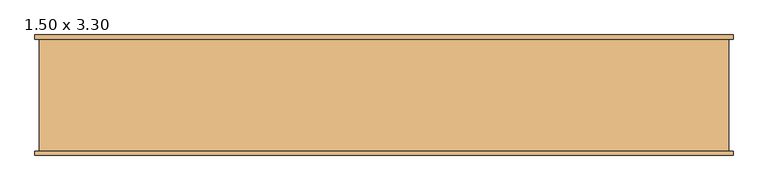
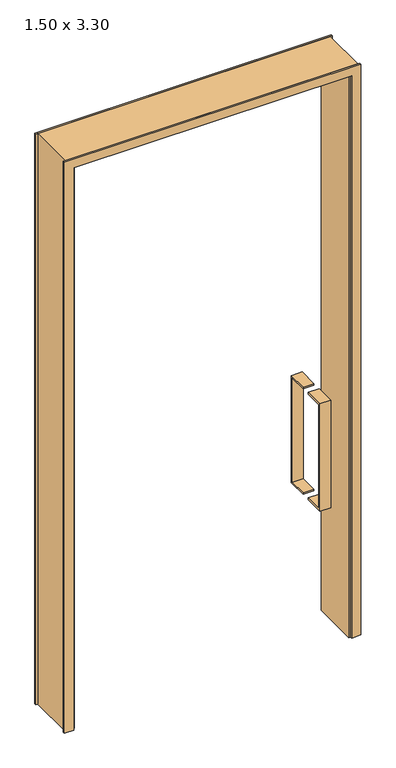
"""IFC4 building model written with IfcOpenShell, lengths in millimetres: door geometry, .CC_ND 300 PORTA PIVOTANTE_COM BANDEIRA_COM EXTENSÃO : 1.50 x 3.30."""

import ifcopenshell
import ifcopenshell.guid

model = None  # the IFC model being written
_history = None  # IfcOwnerHistory: only IFC2X3 demands one
_inside = {}  # id of a spatial element -> (the spatial element, [elements in it])
_under = {}  # id of a project, library or spatial element -> (it, [spatial elements below it])
_declared = {}  # id of a project -> (the project, [libraries it declares])
_typed = {}  # id of a type object -> (the type object, [elements of that type])
_made_of = {}  # id of a material, layer set ... -> (it, [elements and type objects made of it])


def new_model(schema):
    """Start an empty IFC model of exactly this schema.

    Asked for "IFC4X3", IfcOpenShell would pick the latest addendum, in which some entities
    have other attributes; the version numbers below select the first issue.
    IFC2X3 requires an IfcOwnerHistory on every rooted entity: one is made here for all.
    """
    global model, _history
    if schema == "IFC4X3":
        model = ifcopenshell.file(schema_version=(4, 3, 0, 0))
    else:
        model = ifcopenshell.file(schema=schema)
    _inside.clear()
    _under.clear()
    _declared.clear()
    _typed.clear()
    _made_of.clear()
    _history = None
    if model.schema == "IFC2X3":
        org = make("IfcOrganization", Name="unknown")
        user = make(
            "IfcPersonAndOrganization",
            ThePerson=make("IfcPerson", FamilyName="unknown"),
            TheOrganization=org,
        )
        app = make(
            "IfcApplication",
            ApplicationDeveloper=org,
            Version="unknown",
            ApplicationFullName="unknown",
            ApplicationIdentifier="unknown",
        )
        _history = make(
            "IfcOwnerHistory",
            OwningUser=user,
            OwningApplication=app,
            ChangeAction="ADDED",
            CreationDate=0,
        )
    return model


def make(cls, **values):
    """One entity of the class cls with the attributes given. An attribute that is None is left unset."""
    return model.create_entity(
        cls, **{name: value for name, value in values.items() if value is not None}
    )


def rooted(cls, **values):
    """An entity with a GlobalId (a new one), such as an element, a storey or a relation."""
    return make(cls, GlobalId=ifcopenshell.guid.new(), OwnerHistory=_history, **values)


def si_unit(unit_type, name, prefix=None):
    """IfcSIUnit, for example si_unit("LENGTHUNIT", "METRE", prefix="MILLI")."""
    return make("IfcSIUnit", UnitType=unit_type, Prefix=prefix, Name=name)


def assignment(units):
    """IfcUnitAssignment: the units of a project."""
    return None if units is None else make("IfcUnitAssignment", Units=units)


def point(xyz):
    """IfcCartesianPoint."""
    return None if xyz is None else make("IfcCartesianPoint", Coordinates=xyz)


def direction(xyz):
    """IfcDirection."""
    return None if xyz is None else make("IfcDirection", DirectionRatios=xyz)


def frame(location, z_axis=None, x_axis=None):
    """IfcAxis2Placement3D, a coordinate frame: its origin and axes. An axis left out is left unset."""
    return make(
        "IfcAxis2Placement3D",
        Location=point(location),
        Axis=direction(z_axis),
        RefDirection=direction(x_axis),
    )


def origin():
    """The frame at (0, 0, 0) with its axes left unset."""
    return frame((0.0, 0.0, 0.0))


def place(relative_to, where):
    """IfcLocalPlacement: puts the frame where relative to a parent placement (None: the world)."""
    return make(
        "IfcLocalPlacement", PlacementRelTo=relative_to, RelativePlacement=where
    )


def context(
    kind, dimensions, precision=None, world=None, true_north=None, identifier=None
):
    """IfcGeometricRepresentationContext, for example the 3D "Model" context."""
    return make(
        "IfcGeometricRepresentationContext",
        ContextIdentifier=identifier,
        ContextType=kind,
        CoordinateSpaceDimension=dimensions,
        Precision=precision,
        WorldCoordinateSystem=world,
        TrueNorth=true_north,
    )


def project(units=None, contexts=None):
    """IfcProject with its units and contexts."""
    return rooted(
        "IfcProject",
        Name="project",
        RepresentationContexts=contexts,
        UnitsInContext=assignment(units),
    )


def spatial(cls, under=None, at=None, **own):
    """A site, building, storey or space (cls), placed at a placement, below another one or the project."""
    s = rooted(cls, ObjectPlacement=at, **own)
    if under is not None:
        _under.setdefault(under.id(), (under, []))[1].append(s)
    return s


def polyline(points):
    """IfcPolyline through the points."""
    return make("IfcPolyline", Points=[point(p) for p in points])


def outline(outer, holes=None, kind="AREA"):
    """IfcArbitraryClosedProfileDef: a profile drawn as a closed curve; with holes, ...WithVoids."""
    if holes is None:
        return make("IfcArbitraryClosedProfileDef", ProfileType=kind, OuterCurve=outer)
    return make(
        "IfcArbitraryProfileDefWithVoids",
        ProfileType=kind,
        OuterCurve=outer,
        InnerCurves=holes,
    )


def extrude(swept, where, along, depth):
    """IfcExtrudedAreaSolid: the profile swept, set in the frame where, extruded along a direction by depth."""
    return make(
        "IfcExtrudedAreaSolid",
        SweptArea=swept,
        Position=where,
        ExtrudedDirection=direction(along),
        Depth=depth,
    )


def shape(context_of_items, identifier, shape_type, items):
    """IfcShapeRepresentation: the items that make up one representation, for example the "Body"."""
    return make(
        "IfcShapeRepresentation",
        ContextOfItems=context_of_items,
        RepresentationIdentifier=identifier,
        RepresentationType=shape_type,
        Items=items,
    )


def source(mapping_origin, context_of_items, identifier, shape_type, items):
    """IfcRepresentationMap: a shape defined once, which mapped items show again and again."""
    return make(
        "IfcRepresentationMap",
        MappingOrigin=mapping_origin,
        MappedRepresentation=shape(context_of_items, identifier, shape_type, items),
    )


def transform(
    local_origin,
    x_axis=None,
    y_axis=None,
    z_axis=None,
    scale=None,
    scale2=None,
    scale3=None,
    uniform=True,
):
    """IfcCartesianTransformationOperator3D, or its non-uniform kind. x_axis, y_axis, z_axis: its Axis1, 2, 3."""
    if uniform:
        return make(
            "IfcCartesianTransformationOperator3D",
            Axis1=direction(x_axis),
            Axis2=direction(y_axis),
            LocalOrigin=point(local_origin),
            Scale=scale,
            Axis3=direction(z_axis),
        )
    return make(
        "IfcCartesianTransformationOperator3DnonUniform",
        Axis1=direction(x_axis),
        Axis2=direction(y_axis),
        LocalOrigin=point(local_origin),
        Scale=scale,
        Axis3=direction(z_axis),
        Scale2=scale2,
        Scale3=scale3,
    )


def mapped(mapping_source, mapping_target):
    """IfcMappedItem: shows the shape of a source again, moved by a transform."""
    return make(
        "IfcMappedItem", MappingSource=mapping_source, MappingTarget=mapping_target
    )


def made_of(thing, what):
    """Note that an element or type object is made of a material, layer set ...; save() writes the relation."""
    if what is not None:
        _made_of.setdefault(what.id(), (what, []))[1].append(thing)
    return thing


def element(
    cls,
    number,
    at=None,
    inside=None,
    cuts=None,
    type_object=None,
    material=None,
    context=None,
    identifier="Body",
    shape_type=None,
    held_by="IfcProductDefinitionShape",
    body=None,
    shapes=None,
    **own,
):
    """One element of the class cls, such as IfcWall. Its Tag is "e" and its number.

    at: its placement. inside: the storey or other place that contains it. cuts: it is an
    opening in that element (IfcRelVoidsElement). A single representation is given by context,
    identifier, shape_type and body (its items); several are given by shapes. held_by: the class
    of the entity that holds the representations. save() writes the other relations.
    """
    e = rooted(cls, Tag="e%d" % number, ObjectPlacement=at, **own)
    if body is not None:
        shapes = [shape(context, identifier, shape_type, body)]
    if shapes is not None:
        e.Representation = make(held_by, Representations=shapes)
    if inside is not None:
        _inside.setdefault(inside.id(), (inside, []))[1].append(e)
    if cuts is not None:
        rooted(
            "IfcRelVoidsElement", RelatingBuildingElement=cuts, RelatedOpeningElement=e
        )
    if type_object is not None:
        _typed.setdefault(type_object.id(), (type_object, []))[1].append(e)
    return made_of(e, material)


def aggregate(whole, parts):
    """IfcRelAggregates: a whole, such as a stair, and the parts it consists of."""
    return rooted("IfcRelAggregates", RelatingObject=whole, RelatedObjects=parts)


def save(model, path):
    """Write the relations noted so far, then the file.

    IfcRelAggregates (storeys below a building ...), IfcRelContainedInSpatialStructure (elements
    in a storey), IfcRelDefinesByType, IfcRelAssociatesMaterial and IfcRelDeclares: one each for
    every whole, place, type object, material and project.
    """
    for whole, parts in _under.values():
        aggregate(whole, parts)
    for where, things in _inside.values():
        rooted(
            "IfcRelContainedInSpatialStructure",
            RelatedElements=things,
            RelatingStructure=where,
        )
    for kind, things in _typed.values():
        rooted("IfcRelDefinesByType", RelatedObjects=things, RelatingType=kind)
    for what, things in _made_of.values():
        rooted("IfcRelAssociatesMaterial", RelatedObjects=things, RelatingMaterial=what)
    for by, libraries in _declared.values():
        rooted("IfcRelDeclares", RelatingContext=by, RelatedDefinitions=libraries)
    model.write(path)


def door_1_50_x_3_30_2c3f3e4b(model_context):
    return source(origin(), model_context, "Body", "SweptSolid", [
        extrude(outline(polyline([(0.0, -810.0), (0.0, -760.0), (3250.0, -760.0), (3250.0, 760.0), (0.0, 760.0), (0.0, 810.0), (3300.0, 810.0), (3300.0, -810.0), (0.0, -810.0)])), frame((0.0, -139.9, 0.0), z_axis=(0.0, 1.0, 0.0), x_axis=(0.0, 0.0, 1.0)), (0.0, 0.0, 1.0), 10.0),
        extrude(outline(polyline([(0.0, 760.0), (0.0, 810.0), (3300.0, 810.0), (3300.0, -810.0), (0.0, -810.0), (0.0, -760.0), (3250.0, -760.0), (3250.0, 760.0), (0.0, 760.0)])), frame((0.0, 129.9, 0.0), z_axis=(0.0, 1.0, 0.0), x_axis=(0.0, 0.0, 1.0)), (0.0, 0.0, 1.0), 10.0),
        extrude(outline(polyline([(0.0, -800.0), (0.0, -750.0), (3250.0, -750.0), (3250.0, 750.0), (0.0, 750.0), (0.0, 800.0), (3300.0, 800.0), (3300.0, -800.0), (0.0, -800.0)])), frame((0.0, -129.9, 0.0), z_axis=(0.0, 1.0, 0.0), x_axis=(0.0, 0.0, 1.0)), (0.0, 0.0, 1.0), 259.8),
        extrude(outline(polyline([(-25.0, 1410.0), (-25.0, 1400.0), (-125.0, 1400.0), (-125.0, 800.0), (-25.0, 800.0), (-25.0, 790.0), (-135.0, 790.0), (-135.0, 1410.0), (-25.0, 1410.0)])), frame((590.0, 0.0, 0.0), z_axis=(1.0, 0.0, 0.0), x_axis=(0.0, 1.0, 0.0)), (0.0, 0.0, 1.0), 60.0),
        extrude(outline(polyline([(25.0, 1400.0), (25.0, 1410.0), (135.0, 1410.0), (135.0, 790.0), (25.0, 790.0), (25.0, 800.0), (125.0, 800.0), (125.0, 1400.0), (25.0, 1400.0)])), frame((590.0, 0.0, 0.0), z_axis=(1.0, 0.0, 0.0), x_axis=(0.0, 1.0, 0.0)), (0.0, 0.0, 1.0), 60.0),
    ])


if __name__ == "__main__":
    model = new_model("IFC4")
    model_context = context("Model", 3, world=origin())
    ifc_project = project(units=[si_unit("LENGTHUNIT", "METRE", prefix="MILLI")], contexts=[model_context])
    site = spatial("IfcSite", under=ifc_project)
    building = spatial("IfcBuilding", under=site)
    placement = place(None, origin())
    door_1_50_x_3_30_shape = door_1_50_x_3_30_2c3f3e4b(model_context)
    element("IfcDoor", 1, ObjectType=".CC_ND 300 PORTA PIVOTANTE_COM BANDEIRA_COM EXTENSÃO : 1.50 x 3.30", at=placement, inside=building, context=model_context, shape_type="MappedRepresentation", body=[
        mapped(door_1_50_x_3_30_shape, transform((0.0, 0.0, 0.0), x_axis=(1.0, 0.0, 0.0), y_axis=(0.0, 1.0, 0.0), z_axis=(0.0, 0.0, 1.0))),
    ])
    save(model, "model.ifc")

# Revit data of these elements
# Type ".CC_ND 300 PORTA PIVOTANTE_COM BANDEIRA_COM EXTENSÃO : 1.50 x 3.30"
#   Type Mark = "151"
#   Analytic Construction = "<None>"
#   Pivot = 0.10 m
#   Largura moldura = 0.05 m
#   Rough Width = 1.60 m
#   Extensão do acabamento interior [instance default] = 0.00 m
#   Extensão do acabamento exterior [instance default] = 0.00 m
#   Espessura moldura = 0.01 m
#   Espessura batente = 0.05 m
#   Thickness = 0.05 m
#   Rough Height = 3.30 m
#   Altura bandeira = 1.15 m
#   Height = 2.10 m
#   Width = 1.50 m
#   Puxador interno [instance default] = yes
#   Puxador externo [instance default] = yes
#   Número de ripas da porta = 4
#   Moldura interna [instance default] = yes
#   Moldura externa [instance default] = yes
#   Function = 1
#   Puxador = .ALUMÍNIO
#   Porta = .MADEIRA_CEREJEIRA CLARO
#   Moldura = .MADEIRA_CEREJEIRA CLARO
#   Batente = .MADEIRA_CEREJEIRA CLARO
#   Wall Closure = (empty or 0)
# Element 1 (IfcDoor, ".CC_ND 300 PORTA PIVOTANTE_COM BANDEIRA_COM EXTENSÃO : 1.50 x 3.30")
#   Materials on its faces: ".MADEIRA_CEREJEIRA CLARO", ".ALUMÍNIO"
# Materials
#   ".ALUMÍNIO": class "CC_METAIS", colour RGB 244 244 244, transparency 0, Description = "Material alumínio", Cost = 0
#   ".MADEIRA_CEREJEIRA CLARO": class ".CC_MADEIRA REVEST.", colour RGB 233 182 144, transparency 0, Cost = 0
